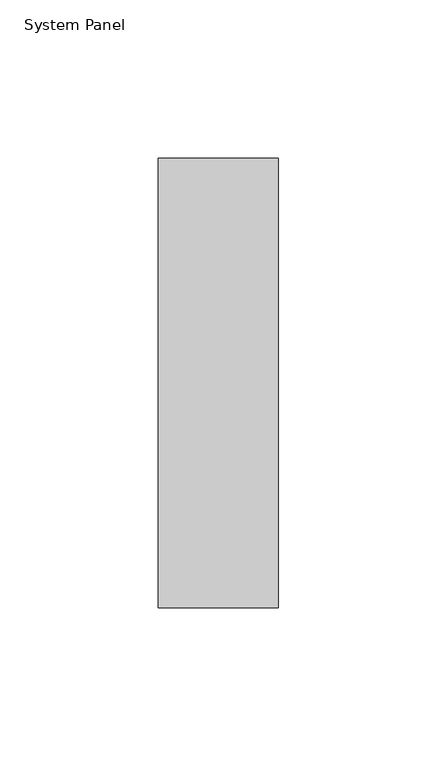
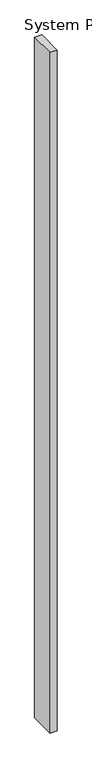
"""IFC4 building model written with IfcOpenShell, lengths in millimetres: plate geometry, System Panel : NLRS_21_CWP_hsb-vulling minerale wol 142 _gen_rsf."""

from ifc_helpers import new_model, si_unit, origin, origin_with_axes, place, context, project, spatial, polyline, outline, extrude, source, transform, mapped, element, save


def system_panel_13b21a00(model_context):
    return source(origin(), model_context, "Body", "SweptSolid", [
        extrude(outline(polyline([(18.9999998, -71.0), (-18.9999998, -71.0), (-18.9999998, 71.0), (18.9999998, 71.0), (18.9999998, -71.0)])), origin_with_axes(), (0.0, 0.0, 1.0), 3849.0),
    ])


if __name__ == "__main__":
    model = new_model("IFC4")
    model_context = context("Model", 3, world=origin())
    ifc_project = project(units=[si_unit("LENGTHUNIT", "METRE", prefix="MILLI")], contexts=[model_context])
    site = spatial("IfcSite", under=ifc_project)
    building = spatial("IfcBuilding", under=site)
    placement = place(None, origin())
    system_panel_shape = system_panel_13b21a00(model_context)
    element("IfcPlate", 1, ObjectType="System Panel : NLRS_21_CWP_hsb-vulling minerale wol 142 _gen_rsf", at=placement, inside=building, context=model_context, shape_type="MappedRepresentation", body=[
        mapped(system_panel_shape, transform((0.0, 0.0, 0.0), x_axis=(1.0, 0.0, 0.0), y_axis=(0.0, 1.0, 0.0), z_axis=(0.0, 0.0, 1.0))),
    ])
    save(model, "model.ifc")

# Revit data of these elements
# Type "System Panel : NLRS_21_CWP_hsb-vulling minerale wol 142 _gen_rsf"
#   Export Type to IFC As = "IfcWall"
#   Type IfcGUID = "07M7mRoiH1CR8m_RSKIwpC"
#   Assembly Code = "21.23"
# Element 1 (IfcPlate, "System Panel : NLRS_21_CWP_hsb-vulling minerale wol 142 _gen_rsf")
#   Materials on its faces: "NLRS_m1_isolatie minerale wol_gen_rsf"
# Materials
#   "NLRS_m1_isolatie minerale wol_gen_rsf": class "M - Anorganische materialen", colour RGB 200 200 140, transparency 0, Keynote = "m1", Manufacturer = "Revit Standards Foundation", URL = "www.revitstandards.org", Description = "isolatie minerale wol", Cost = 0
